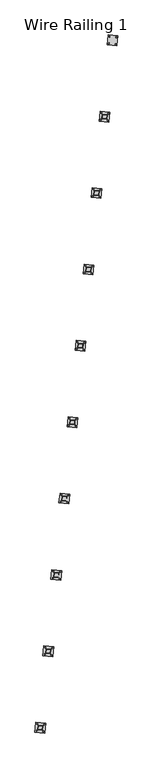
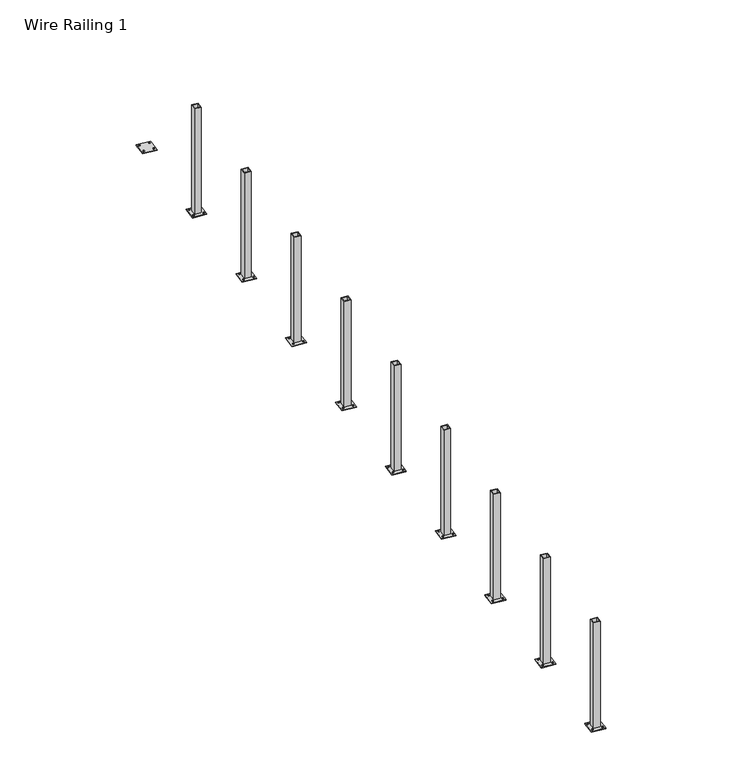
"""IFC4 building model written with IfcOpenShell, lengths in millimetres: railing geometry, Wire Railing 1."""

from ifc_helpers import new_model, si_unit, point, frame, frame_2d, origin, place, context, project, spatial, polyline, circle_curve, trimmed, segment, composite_curve, outline, extrude, source, transform, mapped, element, save


def wire_railing_1_ebebf1ae(model_context):
    return source(origin(), model_context, "Body", "SweptSolid", [
        extrude(outline(composite_curve([segment(trimmed(circle_curve(frame_2d((34190.2063382, 29566.7863564)), 6.35), [point((34196.5215522, 29566.1226006))], [point((34183.8911242, 29567.4501121))], False, "CARTESIAN"), True, "CONTINUOUS"), segment(trimmed(circle_curve(frame_2d((34190.2063382, 29566.7863564)), 6.35), [point((34183.8911242, 29567.4501121))], [point((34196.5215522, 29566.1226006))], False, "CARTESIAN"), True, "CONTINUOUS")], self_intersect=False)), frame((0.0, 0.0, 266395.2), z_axis=(0.0, 0.0, 1.0), x_axis=(1.0, 0.0, 0.0)), (0.0, 0.0, 1.0), 12.7),
        extrude(outline(composite_curve([segment(trimmed(circle_curve(frame_2d((34101.7933417, 29576.0789368)), 6.35), [point((34108.1085557, 29575.415181))], [point((34095.4781277, 29576.7426925))], False, "CARTESIAN"), True, "CONTINUOUS"), segment(trimmed(circle_curve(frame_2d((34101.7933417, 29576.0789368)), 6.35), [point((34095.4781277, 29576.7426925))], [point((34108.1085557, 29575.415181))], False, "CARTESIAN"), True, "CONTINUOUS")], self_intersect=False)), frame((0.0, 0.0, 266395.2), z_axis=(0.0, 0.0, 1.0), x_axis=(1.0, 0.0, 0.0)), (0.0, 0.0, 1.0), 12.7),
        extrude(outline(composite_curve([segment(trimmed(circle_curve(frame_2d((34180.9137578, 29478.3733599)), 6.35), [point((34187.2289719, 29477.7096041))], [point((34174.5985438, 29479.0371156))], False, "CARTESIAN"), True, "CONTINUOUS"), segment(trimmed(circle_curve(frame_2d((34180.9137578, 29478.3733599)), 6.35), [point((34174.5985438, 29479.0371156))], [point((34187.2289719, 29477.7096041))], False, "CARTESIAN"), True, "CONTINUOUS")], self_intersect=False)), frame((0.0, 0.0, 266395.2), z_axis=(0.0, 0.0, 1.0), x_axis=(1.0, 0.0, 0.0)), (0.0, 0.0, 1.0), 12.7),
        extrude(outline(composite_curve([segment(trimmed(circle_curve(frame_2d((34092.5007613, 29487.6659403)), 6.35), [point((34098.8159754, 29487.0021845))], [point((34086.1855473, 29488.329696))], False, "CARTESIAN"), True, "CONTINUOUS"), segment(trimmed(circle_curve(frame_2d((34092.5007613, 29487.6659403)), 6.35), [point((34086.1855473, 29488.329696))], [point((34098.8159754, 29487.0021845))], False, "CARTESIAN"), True, "CONTINUOUS")], self_intersect=False)), frame((0.0, 0.0, 266395.2), z_axis=(0.0, 0.0, 1.0), x_axis=(1.0, 0.0, 0.0)), (0.0, 0.0, 1.0), 12.7),
        extrude(outline(polyline([(34084.8389668, 29597.0158461), (34211.1432475, 29583.7407313), (34197.8681327, 29457.4364505), (34071.563852, 29470.7115654), (34084.8389668, 29597.0158461)])), frame((0.0, 0.0, 266395.2), z_axis=(0.0, 0.0, 1.0), x_axis=(1.0, 0.0, 0.0)), (0.0, 0.0, 1.0), 6.35),
        extrude(outline(polyline([(34114.5091229, 29560.3762548), (34174.5036562, 29554.0705752), (34168.1979767, 29494.0760419), (34108.2034433, 29500.3817214), (34114.5091229, 29560.3762548)]), holes=[polyline([(34120.1605812, 29553.397285), (34115.1824131, 29506.0331797), (34162.5465184, 29501.0550117), (34167.5246864, 29548.4191169), (34120.1605812, 29553.397285)])]), frame((0.0, 0.0, 266395.2), z_axis=(0.0, 0.0, 1.0), x_axis=(1.0, 0.0, 0.0)), (0.0, 0.0, 1.0), 1047.75),
        extrude(outline(composite_curve([segment(trimmed(circle_curve(frame_2d((34293.7976765, 30552.3921032)), 6.35), [point((34300.1128905, 30551.7283474))], [point((34287.4824625, 30553.0558589))], False, "CARTESIAN"), True, "CONTINUOUS"), segment(trimmed(circle_curve(frame_2d((34293.7976765, 30552.3921032)), 6.35), [point((34287.4824625, 30553.0558589))], [point((34300.1128905, 30551.7283474))], False, "CARTESIAN"), True, "CONTINUOUS")], self_intersect=False)), frame((0.0, 0.0, 266395.2), z_axis=(0.0, 0.0, 1.0), x_axis=(1.0, 0.0, 0.0)), (0.0, 0.0, 1.0), 12.7),
        extrude(outline(composite_curve([segment(trimmed(circle_curve(frame_2d((34205.38468, 30561.6846835)), 6.35), [point((34211.699894, 30561.0209278))], [point((34199.069466, 30562.3484393))], False, "CARTESIAN"), True, "CONTINUOUS"), segment(trimmed(circle_curve(frame_2d((34205.38468, 30561.6846835)), 6.35), [point((34199.069466, 30562.3484393))], [point((34211.699894, 30561.0209278))], False, "CARTESIAN"), True, "CONTINUOUS")], self_intersect=False)), frame((0.0, 0.0, 266395.2), z_axis=(0.0, 0.0, 1.0), x_axis=(1.0, 0.0, 0.0)), (0.0, 0.0, 1.0), 12.7),
        extrude(outline(composite_curve([segment(trimmed(circle_curve(frame_2d((34284.5050961, 30463.9791067)), 6.35), [point((34290.8203101, 30463.3153509))], [point((34278.1898821, 30464.6428624))], False, "CARTESIAN"), True, "CONTINUOUS"), segment(trimmed(circle_curve(frame_2d((34284.5050961, 30463.9791067)), 6.35), [point((34278.1898821, 30464.6428624))], [point((34290.8203101, 30463.3153509))], False, "CARTESIAN"), True, "CONTINUOUS")], self_intersect=False)), frame((0.0, 0.0, 266395.2), z_axis=(0.0, 0.0, 1.0), x_axis=(1.0, 0.0, 0.0)), (0.0, 0.0, 1.0), 12.7),
        extrude(outline(composite_curve([segment(trimmed(circle_curve(frame_2d((34196.0920996, 30473.271687)), 6.35), [point((34202.4073136, 30472.6079313))], [point((34189.7768856, 30473.9354428))], False, "CARTESIAN"), True, "CONTINUOUS"), segment(trimmed(circle_curve(frame_2d((34196.0920996, 30473.271687)), 6.35), [point((34189.7768856, 30473.9354428))], [point((34202.4073136, 30472.6079313))], False, "CARTESIAN"), True, "CONTINUOUS")], self_intersect=False)), frame((0.0, 0.0, 266395.2), z_axis=(0.0, 0.0, 1.0), x_axis=(1.0, 0.0, 0.0)), (0.0, 0.0, 1.0), 12.7),
        extrude(outline(polyline([(34188.4303051, 30582.6215929), (34314.7345858, 30569.346478), (34301.459471, 30443.0421973), (34175.1551903, 30456.3173122), (34188.4303051, 30582.6215929)])), frame((0.0, 0.0, 266395.2), z_axis=(0.0, 0.0, 1.0), x_axis=(1.0, 0.0, 0.0)), (0.0, 0.0, 1.0), 6.35),
        extrude(outline(polyline([(34218.1004612, 30545.9820015), (34278.0949945, 30539.676322), (34271.7893149, 30479.6817887), (34211.7947816, 30485.9874682), (34218.1004612, 30545.9820015)]), holes=[polyline([(34223.7519195, 30539.0030318), (34218.7737514, 30491.6389265), (34266.1378567, 30486.6607584), (34271.1160247, 30534.0248637), (34223.7519195, 30539.0030318)])]), frame((0.0, 0.0, 266395.2), z_axis=(0.0, 0.0, 1.0), x_axis=(1.0, 0.0, 0.0)), (0.0, 0.0, 1.0), 1047.75),
        extrude(outline(composite_curve([segment(trimmed(circle_curve(frame_2d((34397.3890148, 31537.9978499)), 6.35), [point((34403.7042288, 31537.3340942))], [point((34391.0738007, 31538.6616057))], False, "CARTESIAN"), True, "CONTINUOUS"), segment(trimmed(circle_curve(frame_2d((34397.3890148, 31537.9978499)), 6.35), [point((34391.0738007, 31538.6616057))], [point((34403.7042288, 31537.3340942))], False, "CARTESIAN"), True, "CONTINUOUS")], self_intersect=False)), frame((0.0, 0.0, 266395.2), z_axis=(0.0, 0.0, 1.0), x_axis=(1.0, 0.0, 0.0)), (0.0, 0.0, 1.0), 12.7),
        extrude(outline(composite_curve([segment(trimmed(circle_curve(frame_2d((34308.9760183, 31547.2904303)), 6.35), [point((34315.2912323, 31546.6266746))], [point((34302.6608042, 31547.9541861))], False, "CARTESIAN"), True, "CONTINUOUS"), segment(trimmed(circle_curve(frame_2d((34308.9760183, 31547.2904303)), 6.35), [point((34302.6608042, 31547.9541861))], [point((34315.2912323, 31546.6266746))], False, "CARTESIAN"), True, "CONTINUOUS")], self_intersect=False)), frame((0.0, 0.0, 266395.2), z_axis=(0.0, 0.0, 1.0), x_axis=(1.0, 0.0, 0.0)), (0.0, 0.0, 1.0), 12.7),
        extrude(outline(composite_curve([segment(trimmed(circle_curve(frame_2d((34388.0964344, 31449.5848534)), 6.35), [point((34394.4116484, 31448.9210977))], [point((34381.7812204, 31450.2486092))], False, "CARTESIAN"), True, "CONTINUOUS"), segment(trimmed(circle_curve(frame_2d((34388.0964344, 31449.5848534)), 6.35), [point((34381.7812204, 31450.2486092))], [point((34394.4116484, 31448.9210977))], False, "CARTESIAN"), True, "CONTINUOUS")], self_intersect=False)), frame((0.0, 0.0, 266395.2), z_axis=(0.0, 0.0, 1.0), x_axis=(1.0, 0.0, 0.0)), (0.0, 0.0, 1.0), 12.7),
        extrude(outline(composite_curve([segment(trimmed(circle_curve(frame_2d((34299.6834379, 31458.8774338)), 6.35), [point((34305.9986519, 31458.2136781))], [point((34293.3682239, 31459.5411896))], False, "CARTESIAN"), True, "CONTINUOUS"), segment(trimmed(circle_curve(frame_2d((34299.6834379, 31458.8774338)), 6.35), [point((34293.3682239, 31459.5411896))], [point((34305.9986519, 31458.2136781))], False, "CARTESIAN"), True, "CONTINUOUS")], self_intersect=False)), frame((0.0, 0.0, 266395.2), z_axis=(0.0, 0.0, 1.0), x_axis=(1.0, 0.0, 0.0)), (0.0, 0.0, 1.0), 12.7),
        extrude(outline(polyline([(34292.0216434, 31568.2273396), (34418.3259241, 31554.9522248), (34405.0508093, 31428.6479441), (34278.7465286, 31441.9230589), (34292.0216434, 31568.2273396)])), frame((0.0, 0.0, 266395.2), z_axis=(0.0, 0.0, 1.0), x_axis=(1.0, 0.0, 0.0)), (0.0, 0.0, 1.0), 6.35),
        extrude(outline(polyline([(34321.6917994, 31531.5877483), (34381.6863328, 31525.2820688), (34375.3806532, 31465.2875354), (34315.3861199, 31471.593215), (34321.6917994, 31531.5877483)]), holes=[polyline([(34327.3432577, 31524.6087785), (34322.3650897, 31477.2446733), (34369.7291949, 31472.2665052), (34374.707363, 31519.6306105), (34327.3432577, 31524.6087785)])]), frame((0.0, 0.0, 266395.2), z_axis=(0.0, 0.0, 1.0), x_axis=(1.0, 0.0, 0.0)), (0.0, 0.0, 1.0), 1047.75),
        extrude(outline(composite_curve([segment(trimmed(circle_curve(frame_2d((34500.9803531, 32523.6035967)), 6.35), [point((34507.2955671, 32522.939841))], [point((34494.665139, 32524.2673525))], False, "CARTESIAN"), True, "CONTINUOUS"), segment(trimmed(circle_curve(frame_2d((34500.9803531, 32523.6035967)), 6.35), [point((34494.665139, 32524.2673525))], [point((34507.2955671, 32522.939841))], False, "CARTESIAN"), True, "CONTINUOUS")], self_intersect=False)), frame((0.0, 0.0, 266395.2), z_axis=(0.0, 0.0, 1.0), x_axis=(1.0, 0.0, 0.0)), (0.0, 0.0, 1.0), 12.7),
        extrude(outline(composite_curve([segment(trimmed(circle_curve(frame_2d((34412.5673566, 32532.8961771)), 6.35), [point((34418.8825706, 32532.2324214))], [point((34406.2521425, 32533.5599328))], False, "CARTESIAN"), True, "CONTINUOUS"), segment(trimmed(circle_curve(frame_2d((34412.5673566, 32532.8961771)), 6.35), [point((34406.2521425, 32533.5599328))], [point((34418.8825706, 32532.2324214))], False, "CARTESIAN"), True, "CONTINUOUS")], self_intersect=False)), frame((0.0, 0.0, 266395.2), z_axis=(0.0, 0.0, 1.0), x_axis=(1.0, 0.0, 0.0)), (0.0, 0.0, 1.0), 12.7),
        extrude(outline(composite_curve([segment(trimmed(circle_curve(frame_2d((34491.6877727, 32435.1906002)), 6.35), [point((34498.0029867, 32434.5268445))], [point((34485.3725587, 32435.854356))], False, "CARTESIAN"), True, "CONTINUOUS"), segment(trimmed(circle_curve(frame_2d((34491.6877727, 32435.1906002)), 6.35), [point((34485.3725587, 32435.854356))], [point((34498.0029867, 32434.5268445))], False, "CARTESIAN"), True, "CONTINUOUS")], self_intersect=False)), frame((0.0, 0.0, 266395.2), z_axis=(0.0, 0.0, 1.0), x_axis=(1.0, 0.0, 0.0)), (0.0, 0.0, 1.0), 12.7),
        extrude(outline(composite_curve([segment(trimmed(circle_curve(frame_2d((34403.2747762, 32444.4831806)), 6.35), [point((34409.5899902, 32443.8194249))], [point((34396.9595622, 32445.1469363))], False, "CARTESIAN"), True, "CONTINUOUS"), segment(trimmed(circle_curve(frame_2d((34403.2747762, 32444.4831806)), 6.35), [point((34396.9595622, 32445.1469363))], [point((34409.5899902, 32443.8194249))], False, "CARTESIAN"), True, "CONTINUOUS")], self_intersect=False)), frame((0.0, 0.0, 266395.2), z_axis=(0.0, 0.0, 1.0), x_axis=(1.0, 0.0, 0.0)), (0.0, 0.0, 1.0), 12.7),
        extrude(outline(polyline([(34395.6129817, 32553.8330864), (34521.9172624, 32540.5579716), (34508.6421476, 32414.2536909), (34382.3378669, 32427.5288057), (34395.6129817, 32553.8330864)])), frame((0.0, 0.0, 266395.2), z_axis=(0.0, 0.0, 1.0), x_axis=(1.0, 0.0, 0.0)), (0.0, 0.0, 1.0), 6.35),
        extrude(outline(polyline([(34425.2831377, 32517.1934951), (34485.2776711, 32510.8878156), (34478.9719915, 32450.8932822), (34418.9774582, 32457.1989618), (34425.2831377, 32517.1934951)]), holes=[polyline([(34430.934596, 32510.2145253), (34425.956428, 32462.8504201), (34473.3205332, 32457.872252), (34478.2987013, 32505.2363573), (34430.934596, 32510.2145253)])]), frame((0.0, 0.0, 266395.2), z_axis=(0.0, 0.0, 1.0), x_axis=(1.0, 0.0, 0.0)), (0.0, 0.0, 1.0), 1047.75),
        extrude(outline(composite_curve([segment(trimmed(circle_curve(frame_2d((34604.5716914, 33509.2093435)), 6.35), [point((34610.8869054, 33508.5455877))], [point((34598.2564773, 33509.8730992))], False, "CARTESIAN"), True, "CONTINUOUS"), segment(trimmed(circle_curve(frame_2d((34604.5716914, 33509.2093435)), 6.35), [point((34598.2564773, 33509.8730992))], [point((34610.8869054, 33508.5455877))], False, "CARTESIAN"), True, "CONTINUOUS")], self_intersect=False)), frame((0.0, 0.0, 266395.2), z_axis=(0.0, 0.0, 1.0), x_axis=(1.0, 0.0, 0.0)), (0.0, 0.0, 1.0), 12.7),
        extrude(outline(composite_curve([segment(trimmed(circle_curve(frame_2d((34516.1586949, 33518.5019239)), 6.35), [point((34522.4739089, 33517.8381681))], [point((34509.8434808, 33519.1656796))], False, "CARTESIAN"), True, "CONTINUOUS"), segment(trimmed(circle_curve(frame_2d((34516.1586949, 33518.5019239)), 6.35), [point((34509.8434808, 33519.1656796))], [point((34522.4739089, 33517.8381681))], False, "CARTESIAN"), True, "CONTINUOUS")], self_intersect=False)), frame((0.0, 0.0, 266395.2), z_axis=(0.0, 0.0, 1.0), x_axis=(1.0, 0.0, 0.0)), (0.0, 0.0, 1.0), 12.7),
        extrude(outline(composite_curve([segment(trimmed(circle_curve(frame_2d((34595.279111, 33420.796347)), 6.35), [point((34601.594325, 33420.1325913))], [point((34588.9638969, 33421.4601027))], False, "CARTESIAN"), True, "CONTINUOUS"), segment(trimmed(circle_curve(frame_2d((34595.279111, 33420.796347)), 6.35), [point((34588.9638969, 33421.4601027))], [point((34601.594325, 33420.1325913))], False, "CARTESIAN"), True, "CONTINUOUS")], self_intersect=False)), frame((0.0, 0.0, 266395.2), z_axis=(0.0, 0.0, 1.0), x_axis=(1.0, 0.0, 0.0)), (0.0, 0.0, 1.0), 12.7),
        extrude(outline(composite_curve([segment(trimmed(circle_curve(frame_2d((34506.8661145, 33430.0889274)), 6.35), [point((34513.1813285, 33429.4251716))], [point((34500.5509004, 33430.7526831))], False, "CARTESIAN"), True, "CONTINUOUS"), segment(trimmed(circle_curve(frame_2d((34506.8661145, 33430.0889274)), 6.35), [point((34500.5509004, 33430.7526831))], [point((34513.1813285, 33429.4251716))], False, "CARTESIAN"), True, "CONTINUOUS")], self_intersect=False)), frame((0.0, 0.0, 266395.2), z_axis=(0.0, 0.0, 1.0), x_axis=(1.0, 0.0, 0.0)), (0.0, 0.0, 1.0), 12.7),
        extrude(outline(polyline([(34499.20432, 33539.4388332), (34625.5086007, 33526.1637184), (34612.2334859, 33399.8594377), (34485.9292051, 33413.1345525), (34499.20432, 33539.4388332)])), frame((0.0, 0.0, 266395.2), z_axis=(0.0, 0.0, 1.0), x_axis=(1.0, 0.0, 0.0)), (0.0, 0.0, 1.0), 6.35),
        extrude(outline(polyline([(34528.874476, 33502.7992419), (34588.8690094, 33496.4935623), (34582.5633298, 33436.499029), (34522.5687965, 33442.8047085), (34528.874476, 33502.7992419)]), holes=[polyline([(34534.5259343, 33495.8202721), (34529.5477663, 33448.4561668), (34576.9118715, 33443.4779988), (34581.8900396, 33490.842104), (34534.5259343, 33495.8202721)])]), frame((0.0, 0.0, 266395.2), z_axis=(0.0, 0.0, 1.0), x_axis=(1.0, 0.0, 0.0)), (0.0, 0.0, 1.0), 1047.75),
        extrude(outline(composite_curve([segment(trimmed(circle_curve(frame_2d((34708.1630296, 34494.8150903)), 6.35), [point((34714.4782437, 34494.1513345))], [point((34701.8478156, 34495.478846))], False, "CARTESIAN"), True, "CONTINUOUS"), segment(trimmed(circle_curve(frame_2d((34708.1630296, 34494.8150903)), 6.35), [point((34701.8478156, 34495.478846))], [point((34714.4782437, 34494.1513345))], False, "CARTESIAN"), True, "CONTINUOUS")], self_intersect=False)), frame((0.0, 0.0, 266395.2), z_axis=(0.0, 0.0, 1.0), x_axis=(1.0, 0.0, 0.0)), (0.0, 0.0, 1.0), 12.7),
        extrude(outline(composite_curve([segment(trimmed(circle_curve(frame_2d((34619.7500332, 34504.1076707)), 6.35), [point((34626.0652472, 34503.4439149))], [point((34613.4348191, 34504.7714264))], False, "CARTESIAN"), True, "CONTINUOUS"), segment(trimmed(circle_curve(frame_2d((34619.7500332, 34504.1076707)), 6.35), [point((34613.4348191, 34504.7714264))], [point((34626.0652472, 34503.4439149))], False, "CARTESIAN"), True, "CONTINUOUS")], self_intersect=False)), frame((0.0, 0.0, 266395.2), z_axis=(0.0, 0.0, 1.0), x_axis=(1.0, 0.0, 0.0)), (0.0, 0.0, 1.0), 12.7),
        extrude(outline(composite_curve([segment(trimmed(circle_curve(frame_2d((34698.8704493, 34406.4020938)), 6.35), [point((34705.1856633, 34405.738338))], [point((34692.5552352, 34407.0658495))], False, "CARTESIAN"), True, "CONTINUOUS"), segment(trimmed(circle_curve(frame_2d((34698.8704493, 34406.4020938)), 6.35), [point((34692.5552352, 34407.0658495))], [point((34705.1856633, 34405.738338))], False, "CARTESIAN"), True, "CONTINUOUS")], self_intersect=False)), frame((0.0, 0.0, 266395.2), z_axis=(0.0, 0.0, 1.0), x_axis=(1.0, 0.0, 0.0)), (0.0, 0.0, 1.0), 12.7),
        extrude(outline(composite_curve([segment(trimmed(circle_curve(frame_2d((34610.4574528, 34415.6946742)), 6.35), [point((34616.7726668, 34415.0309184))], [point((34604.1422387, 34416.3584299))], False, "CARTESIAN"), True, "CONTINUOUS"), segment(trimmed(circle_curve(frame_2d((34610.4574528, 34415.6946742)), 6.35), [point((34604.1422387, 34416.3584299))], [point((34616.7726668, 34415.0309184))], False, "CARTESIAN"), True, "CONTINUOUS")], self_intersect=False)), frame((0.0, 0.0, 266395.2), z_axis=(0.0, 0.0, 1.0), x_axis=(1.0, 0.0, 0.0)), (0.0, 0.0, 1.0), 12.7),
        extrude(outline(polyline([(34602.7956583, 34525.04458), (34729.099939, 34511.7694652), (34715.8248241, 34385.4651844), (34589.5205434, 34398.7402993), (34602.7956583, 34525.04458)])), frame((0.0, 0.0, 266395.2), z_axis=(0.0, 0.0, 1.0), x_axis=(1.0, 0.0, 0.0)), (0.0, 0.0, 1.0), 6.35),
        extrude(outline(polyline([(34632.4658143, 34488.4049887), (34692.4603476, 34482.0993091), (34686.1546681, 34422.1047758), (34626.1601348, 34428.4104553), (34632.4658143, 34488.4049887)]), holes=[polyline([(34638.1172726, 34481.4260189), (34633.1391045, 34434.0619136), (34680.5032098, 34429.0837455), (34685.4813779, 34476.4478508), (34638.1172726, 34481.4260189)])]), frame((0.0, 0.0, 266395.2), z_axis=(0.0, 0.0, 1.0), x_axis=(1.0, 0.0, 0.0)), (0.0, 0.0, 1.0), 1047.75),
        extrude(outline(composite_curve([segment(trimmed(circle_curve(frame_2d((34811.7543679, 35480.4208371)), 6.35), [point((34818.069582, 35479.7570813))], [point((34805.4391539, 35481.0845928))], False, "CARTESIAN"), True, "CONTINUOUS"), segment(trimmed(circle_curve(frame_2d((34811.7543679, 35480.4208371)), 6.35), [point((34805.4391539, 35481.0845928))], [point((34818.069582, 35479.7570813))], False, "CARTESIAN"), True, "CONTINUOUS")], self_intersect=False)), frame((0.0, 0.0, 266395.2), z_axis=(0.0, 0.0, 1.0), x_axis=(1.0, 0.0, 0.0)), (0.0, 0.0, 1.0), 12.7),
        extrude(outline(composite_curve([segment(trimmed(circle_curve(frame_2d((34723.3413714, 35489.7134174)), 6.35), [point((34729.6565855, 35489.0496617))], [point((34717.0261574, 35490.3771732))], False, "CARTESIAN"), True, "CONTINUOUS"), segment(trimmed(circle_curve(frame_2d((34723.3413714, 35489.7134174)), 6.35), [point((34717.0261574, 35490.3771732))], [point((34729.6565855, 35489.0496617))], False, "CARTESIAN"), True, "CONTINUOUS")], self_intersect=False)), frame((0.0, 0.0, 266395.2), z_axis=(0.0, 0.0, 1.0), x_axis=(1.0, 0.0, 0.0)), (0.0, 0.0, 1.0), 12.7),
        extrude(outline(composite_curve([segment(trimmed(circle_curve(frame_2d((34802.4617876, 35392.0078406)), 6.35), [point((34808.7770016, 35391.3440848))], [point((34796.1465735, 35392.6715963))], False, "CARTESIAN"), True, "CONTINUOUS"), segment(trimmed(circle_curve(frame_2d((34802.4617876, 35392.0078406)), 6.35), [point((34796.1465735, 35392.6715963))], [point((34808.7770016, 35391.3440848))], False, "CARTESIAN"), True, "CONTINUOUS")], self_intersect=False)), frame((0.0, 0.0, 266395.2), z_axis=(0.0, 0.0, 1.0), x_axis=(1.0, 0.0, 0.0)), (0.0, 0.0, 1.0), 12.7),
        extrude(outline(composite_curve([segment(trimmed(circle_curve(frame_2d((34714.0487911, 35401.3004209)), 6.35), [point((34720.3640051, 35400.6366652))], [point((34707.733577, 35401.9641767))], False, "CARTESIAN"), True, "CONTINUOUS"), segment(trimmed(circle_curve(frame_2d((34714.0487911, 35401.3004209)), 6.35), [point((34707.733577, 35401.9641767))], [point((34720.3640051, 35400.6366652))], False, "CARTESIAN"), True, "CONTINUOUS")], self_intersect=False)), frame((0.0, 0.0, 266395.2), z_axis=(0.0, 0.0, 1.0), x_axis=(1.0, 0.0, 0.0)), (0.0, 0.0, 1.0), 12.7),
        extrude(outline(polyline([(34706.3869966, 35510.6503268), (34832.6912773, 35497.3752119), (34819.4161624, 35371.0709312), (34693.1118817, 35384.3460461), (34706.3869966, 35510.6503268)])), frame((0.0, 0.0, 266395.2), z_axis=(0.0, 0.0, 1.0), x_axis=(1.0, 0.0, 0.0)), (0.0, 0.0, 1.0), 6.35),
        extrude(outline(polyline([(34736.0571526, 35474.0107354), (34796.0516859, 35467.7050559), (34789.7460064, 35407.7105226), (34729.7514731, 35414.0162021), (34736.0571526, 35474.0107354)]), holes=[polyline([(34741.7086109, 35467.0317657), (34736.7304428, 35419.6676604), (34784.0945481, 35414.6894923), (34789.0727162, 35462.0535976), (34741.7086109, 35467.0317657)])]), frame((0.0, 0.0, 266395.2), z_axis=(0.0, 0.0, 1.0), x_axis=(1.0, 0.0, 0.0)), (0.0, 0.0, 1.0), 1047.75),
        extrude(outline(composite_curve([segment(trimmed(circle_curve(frame_2d((34915.3457062, 36466.0265838)), 6.35), [point((34921.6609203, 36465.3628281))], [point((34909.0304922, 36466.6903396))], False, "CARTESIAN"), True, "CONTINUOUS"), segment(trimmed(circle_curve(frame_2d((34915.3457062, 36466.0265838)), 6.35), [point((34909.0304922, 36466.6903396))], [point((34921.6609203, 36465.3628281))], False, "CARTESIAN"), True, "CONTINUOUS")], self_intersect=False)), frame((0.0, 0.0, 266395.2), z_axis=(0.0, 0.0, 1.0), x_axis=(1.0, 0.0, 0.0)), (0.0, 0.0, 1.0), 12.7),
        extrude(outline(composite_curve([segment(trimmed(circle_curve(frame_2d((34826.9327097, 36475.3191642)), 6.35), [point((34833.2479238, 36474.6554085))], [point((34820.6174957, 36475.98292))], False, "CARTESIAN"), True, "CONTINUOUS"), segment(trimmed(circle_curve(frame_2d((34826.9327097, 36475.3191642)), 6.35), [point((34820.6174957, 36475.98292))], [point((34833.2479238, 36474.6554085))], False, "CARTESIAN"), True, "CONTINUOUS")], self_intersect=False)), frame((0.0, 0.0, 266395.2), z_axis=(0.0, 0.0, 1.0), x_axis=(1.0, 0.0, 0.0)), (0.0, 0.0, 1.0), 12.7),
        extrude(outline(composite_curve([segment(trimmed(circle_curve(frame_2d((34906.0531258, 36377.6135873)), 6.35), [point((34912.3683399, 36376.9498316))], [point((34899.7379118, 36378.2773431))], False, "CARTESIAN"), True, "CONTINUOUS"), segment(trimmed(circle_curve(frame_2d((34906.0531258, 36377.6135873)), 6.35), [point((34899.7379118, 36378.2773431))], [point((34912.3683399, 36376.9498316))], False, "CARTESIAN"), True, "CONTINUOUS")], self_intersect=False)), frame((0.0, 0.0, 266395.2), z_axis=(0.0, 0.0, 1.0), x_axis=(1.0, 0.0, 0.0)), (0.0, 0.0, 1.0), 12.7),
        extrude(outline(composite_curve([segment(trimmed(circle_curve(frame_2d((34817.6401293, 36386.9061677)), 6.35), [point((34823.9553434, 36386.242412))], [point((34811.3249153, 36387.5699235))], False, "CARTESIAN"), True, "CONTINUOUS"), segment(trimmed(circle_curve(frame_2d((34817.6401293, 36386.9061677)), 6.35), [point((34811.3249153, 36387.5699235))], [point((34823.9553434, 36386.242412))], False, "CARTESIAN"), True, "CONTINUOUS")], self_intersect=False)), frame((0.0, 0.0, 266395.2), z_axis=(0.0, 0.0, 1.0), x_axis=(1.0, 0.0, 0.0)), (0.0, 0.0, 1.0), 12.7),
        extrude(outline(polyline([(34809.9783348, 36496.2560735), (34936.2826156, 36482.9809587), (34923.0075007, 36356.676678), (34796.70322, 36369.9517928), (34809.9783348, 36496.2560735)])), frame((0.0, 0.0, 266395.2), z_axis=(0.0, 0.0, 1.0), x_axis=(1.0, 0.0, 0.0)), (0.0, 0.0, 1.0), 6.35),
        extrude(outline(polyline([(34839.6484909, 36459.6164822), (34899.6430242, 36453.3108027), (34893.3373447, 36393.3162693), (34833.3428113, 36399.6219489), (34839.6484909, 36459.6164822)]), holes=[polyline([(34845.2999492, 36452.6375124), (34840.3217811, 36405.2734072), (34887.6858864, 36400.2952391), (34892.6640544, 36447.6593444), (34845.2999492, 36452.6375124)])]), frame((0.0, 0.0, 266395.2), z_axis=(0.0, 0.0, 1.0), x_axis=(1.0, 0.0, 0.0)), (0.0, 0.0, 1.0), 1047.75),
        extrude(outline(composite_curve([segment(trimmed(circle_curve(frame_2d((35018.9370445, 37451.6323306)), 6.35), [point((35025.2522586, 37450.9685749))], [point((35012.6218305, 37452.2960864))], False, "CARTESIAN"), True, "CONTINUOUS"), segment(trimmed(circle_curve(frame_2d((35018.9370445, 37451.6323306)), 6.35), [point((35012.6218305, 37452.2960864))], [point((35025.2522586, 37450.9685749))], False, "CARTESIAN"), True, "CONTINUOUS")], self_intersect=False)), frame((0.0, 0.0, 266395.2), z_axis=(0.0, 0.0, 1.0), x_axis=(1.0, 0.0, 0.0)), (0.0, 0.0, 1.0), 12.7),
        extrude(outline(composite_curve([segment(trimmed(circle_curve(frame_2d((34930.524048, 37460.924911)), 6.35), [point((34936.8392621, 37460.2611553))], [point((34924.208834, 37461.5886667))], False, "CARTESIAN"), True, "CONTINUOUS"), segment(trimmed(circle_curve(frame_2d((34930.524048, 37460.924911)), 6.35), [point((34924.208834, 37461.5886667))], [point((34936.8392621, 37460.2611553))], False, "CARTESIAN"), True, "CONTINUOUS")], self_intersect=False)), frame((0.0, 0.0, 266395.2), z_axis=(0.0, 0.0, 1.0), x_axis=(1.0, 0.0, 0.0)), (0.0, 0.0, 1.0), 12.7),
        extrude(outline(composite_curve([segment(trimmed(circle_curve(frame_2d((35009.6444641, 37363.2193341)), 6.35), [point((35015.9596782, 37362.5555784))], [point((35003.3292501, 37363.8830899))], False, "CARTESIAN"), True, "CONTINUOUS"), segment(trimmed(circle_curve(frame_2d((35009.6444641, 37363.2193341)), 6.35), [point((35003.3292501, 37363.8830899))], [point((35015.9596782, 37362.5555784))], False, "CARTESIAN"), True, "CONTINUOUS")], self_intersect=False)), frame((0.0, 0.0, 266395.2), z_axis=(0.0, 0.0, 1.0), x_axis=(1.0, 0.0, 0.0)), (0.0, 0.0, 1.0), 12.7),
        extrude(outline(composite_curve([segment(trimmed(circle_curve(frame_2d((34921.2314676, 37372.5119145)), 6.35), [point((34927.5466817, 37371.8481588))], [point((34914.9162536, 37373.1756702))], False, "CARTESIAN"), True, "CONTINUOUS"), segment(trimmed(circle_curve(frame_2d((34921.2314676, 37372.5119145)), 6.35), [point((34914.9162536, 37373.1756702))], [point((34927.5466817, 37371.8481588))], False, "CARTESIAN"), True, "CONTINUOUS")], self_intersect=False)), frame((0.0, 0.0, 266395.2), z_axis=(0.0, 0.0, 1.0), x_axis=(1.0, 0.0, 0.0)), (0.0, 0.0, 1.0), 12.7),
        extrude(outline(polyline([(34913.5696731, 37481.8618203), (35039.8739538, 37468.5867055), (35026.598839, 37342.2824248), (34900.2945583, 37355.5575396), (34913.5696731, 37481.8618203)])), frame((0.0, 0.0, 266395.2), z_axis=(0.0, 0.0, 1.0), x_axis=(1.0, 0.0, 0.0)), (0.0, 0.0, 1.0), 6.35),
        extrude(outline(polyline([(34943.2398292, 37445.222229), (35003.2343625, 37438.9165494), (34996.928683, 37378.9220161), (34936.9341496, 37385.2276957), (34943.2398292, 37445.222229)]), holes=[polyline([(34948.8912875, 37438.2432592), (34943.9131194, 37390.879154), (34991.2772247, 37385.9009859), (34996.2553927, 37433.2650912), (34948.8912875, 37438.2432592)])]), frame((0.0, 0.0, 266395.2), z_axis=(0.0, 0.0, 1.0), x_axis=(1.0, 0.0, 0.0)), (0.0, 0.0, 1.0), 1047.75),
        extrude(outline(composite_curve([segment(trimmed(circle_curve(frame_2d((35122.5283828, 38437.2380774)), 6.35), [point((35128.8435968, 38436.5743216))], [point((35116.2131688, 38437.9018331))], False, "CARTESIAN"), True, "CONTINUOUS"), segment(trimmed(circle_curve(frame_2d((35122.5283828, 38437.2380774)), 6.35), [point((35116.2131688, 38437.9018331))], [point((35128.8435968, 38436.5743216))], False, "CARTESIAN"), True, "CONTINUOUS")], self_intersect=False)), frame((0.0, 0.0, 266395.2), z_axis=(0.0, 0.0, 1.0), x_axis=(1.0, 0.0, 0.0)), (0.0, 0.0, 1.0), 12.7),
        extrude(outline(composite_curve([segment(trimmed(circle_curve(frame_2d((35034.1153863, 38446.5306578)), 6.35), [point((35040.4306003, 38445.866902))], [point((35027.8001723, 38447.1944135))], False, "CARTESIAN"), True, "CONTINUOUS"), segment(trimmed(circle_curve(frame_2d((35034.1153863, 38446.5306578)), 6.35), [point((35027.8001723, 38447.1944135))], [point((35040.4306003, 38445.866902))], False, "CARTESIAN"), True, "CONTINUOUS")], self_intersect=False)), frame((0.0, 0.0, 266395.2), z_axis=(0.0, 0.0, 1.0), x_axis=(1.0, 0.0, 0.0)), (0.0, 0.0, 1.0), 12.7),
        extrude(outline(composite_curve([segment(trimmed(circle_curve(frame_2d((35113.2358024, 38348.8250809)), 6.35), [point((35119.5510165, 38348.1613251))], [point((35106.9205884, 38349.4888366))], False, "CARTESIAN"), True, "CONTINUOUS"), segment(trimmed(circle_curve(frame_2d((35113.2358024, 38348.8250809)), 6.35), [point((35106.9205884, 38349.4888366))], [point((35119.5510165, 38348.1613251))], False, "CARTESIAN"), True, "CONTINUOUS")], self_intersect=False)), frame((0.0, 0.0, 266395.2), z_axis=(0.0, 0.0, 1.0), x_axis=(1.0, 0.0, 0.0)), (0.0, 0.0, 1.0), 12.7),
        extrude(outline(composite_curve([segment(trimmed(circle_curve(frame_2d((35024.8228059, 38358.1176613)), 6.35), [point((35031.13802, 38357.4539055))], [point((35018.5075919, 38358.781417))], False, "CARTESIAN"), True, "CONTINUOUS"), segment(trimmed(circle_curve(frame_2d((35024.8228059, 38358.1176613)), 6.35), [point((35018.5075919, 38358.781417))], [point((35031.13802, 38357.4539055))], False, "CARTESIAN"), True, "CONTINUOUS")], self_intersect=False)), frame((0.0, 0.0, 266395.2), z_axis=(0.0, 0.0, 1.0), x_axis=(1.0, 0.0, 0.0)), (0.0, 0.0, 1.0), 12.7),
        extrude(outline(polyline([(35017.1610114, 38467.4675671), (35143.4652921, 38454.1924523), (35130.1901773, 38327.8881716), (35003.8858966, 38341.1632864), (35017.1610114, 38467.4675671)])), frame((0.0, 0.0, 266395.2), z_axis=(0.0, 0.0, 1.0), x_axis=(1.0, 0.0, 0.0)), (0.0, 0.0, 1.0), 6.35),
    ])


if __name__ == "__main__":
    model = new_model("IFC4")
    model_context = context("Model", 3, world=origin())
    ifc_project = project(units=[si_unit("LENGTHUNIT", "METRE", prefix="MILLI")], contexts=[model_context])
    site = spatial("IfcSite", under=ifc_project)
    building = spatial("IfcBuilding", under=site)
    placement = place(None, origin())
    wire_railing_1_shape = wire_railing_1_ebebf1ae(model_context)
    element("IfcRailing", 1, ObjectType="Wire Railing 1", at=placement, inside=building, context=model_context, shape_type="MappedRepresentation", body=[
        mapped(wire_railing_1_shape, transform((0.0, 0.0, 0.0), x_axis=(1.0, 0.0, 0.0), y_axis=(0.0, 1.0, 0.0), z_axis=(0.0, 0.0, 1.0))),
    ])
    save(model, "model.ifc")

# Revit data of these elements
# Element 1 (IfcRailing, "Wire Railing 1")
#   Materials on its faces: "2 1/2\" X 2 1/2\" ALUM. SQUARE POST (38\" O.C. MAX)", "WIRE RAILING (3\" O.C.)", "ALUM. PLATE TOP RAIL"
# Materials
#   "2 1/2\" X 2 1/2\" ALUM. SQUARE POST (38\" O.C. MAX)": class "Metal", colour RGB 244 244 244, transparency 0, Manufacturer = "Kawneer", URL = "http://www.kawneer.com/kawneer/north_america/en/home.asp", Cost = 0
#   "WIRE RAILING (3\" O.C.)": class "Metal", colour RGB 244 244 244, transparency 0, Manufacturer = "Kawneer", URL = "http://www.kawneer.com/kawneer/north_america/en/home.asp", Cost = 0
#   "ALUM. PLATE TOP RAIL": class "Metal", colour RGB 244 244 244, transparency 0, Manufacturer = "Kawneer", URL = "http://www.kawneer.com/kawneer/north_america/en/home.asp", Cost = 0
